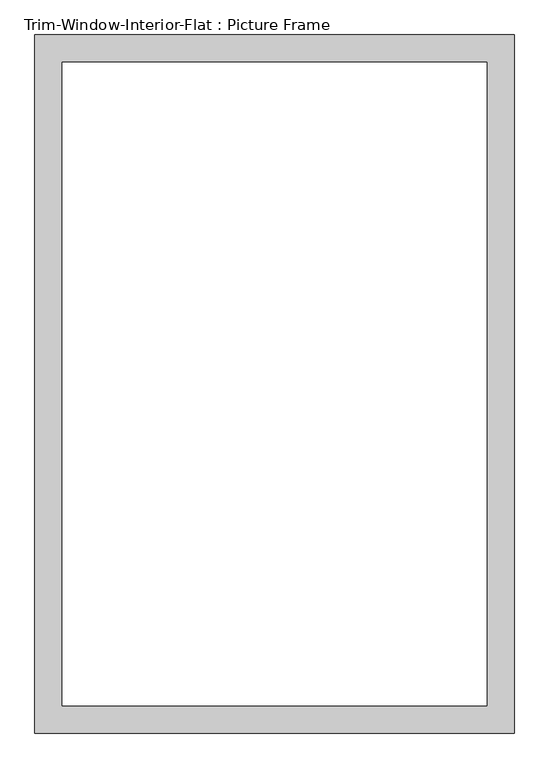
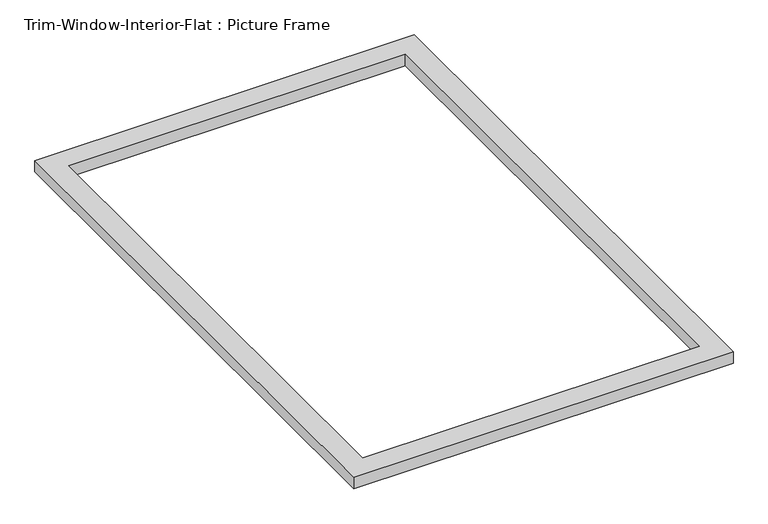
"""IFC4 building model written with IfcOpenShell, lengths in millimetres: proxy geometry, Trim-Window-Interior-Flat : Picture Frame."""

from ifc_helpers import new_model, si_unit, origin, origin_with_axes, place, context, project, spatial, polyline, outline, extrude, source, transform, mapped, element, save


def trim_window_interior_flat_picture_frame_edb5e600(model_context):
    return source(origin(), model_context, "Body", "SweptSolid", [
        extrude(outline(polyline([(501.65, 44.45), (501.65, -1416.05), (-501.65, -1416.05), (-501.65, 44.45), (501.65, 44.45)]), holes=[polyline([(444.5, -12.7), (-444.5, -12.7), (-444.5, -1358.9), (444.5, -1358.9), (444.5, -12.7)])]), origin_with_axes(), (0.0, 0.0, 1.0), 31.75),
    ])


if __name__ == "__main__":
    model = new_model("IFC4")
    model_context = context("Model", 3, world=origin())
    ifc_project = project(units=[si_unit("LENGTHUNIT", "METRE", prefix="MILLI")], contexts=[model_context])
    site = spatial("IfcSite", under=ifc_project)
    building = spatial("IfcBuilding", under=site)
    placement = place(None, origin())
    trim_window_interior_flat_picture_frame_shape = trim_window_interior_flat_picture_frame_edb5e600(model_context)
    element("IfcBuildingElementProxy", 1, Name="Trim-Window-Interior-Flat : Picture Frame", ObjectType="Trim-Window-Interior-Flat : Picture Frame", at=placement, inside=building, context=model_context, shape_type="MappedRepresentation", body=[
        mapped(trim_window_interior_flat_picture_frame_shape, transform((0.0, 0.0, 0.0), x_axis=(1.0, 0.0, 0.0), y_axis=(0.0, 1.0, 0.0), z_axis=(0.0, 0.0, 1.0))),
    ])
    save(model, "model.ifc")

# Revit data of these elements
# Type "Trim-Window-Interior-Flat : Picture Frame"
#   Trim Thickness_Picture Frame = 0' - 1 1/4"
#   Trim Width = 0' - 2 1/4"
#   Trim Thickness_with Sill = 0' - 0 3/4"
#   Sill Thickness = 0' - 1 1/4"
#   Opening Width [instance default] = 2' - 0"
#   Opening Height [instance default] = 3' - 0"
#   Default Elevation = 4' - 0"
#   Sill = no
#   Picture Frame = yes
#   Trim Material [instance default] = none
# Element 1 (IfcBuildingElementProxy, "Trim-Window-Interior-Flat : Picture Frame")
#   Opening Width = 3' - 0"
#   Opening Height = 4' - 6"
#   Trim Material = Maple - Semigloss(Rotated)
#   Materials on its faces: "Maple - Semigloss(Rotated)"
# Materials
#   "Maple - Semigloss(Rotated)": class "Wood", colour RGB 196 161 118, transparency 0, Description = "Acer Saccharum", Cost = 0
